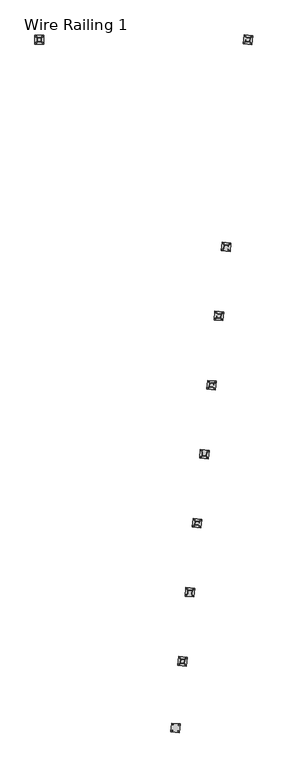
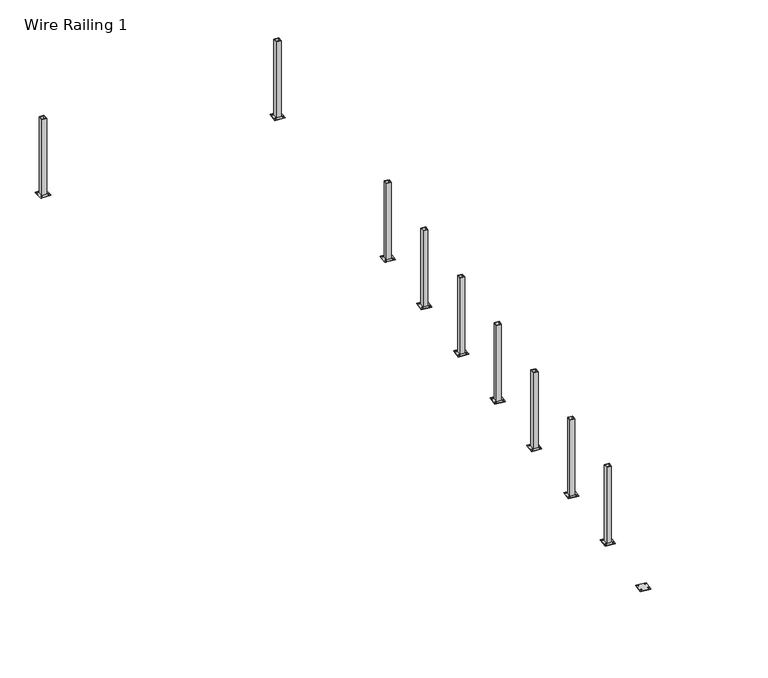
"""IFC4 building model written with IfcOpenShell, lengths in millimetres: railing geometry, Wire Railing 1."""

from ifc_helpers import new_model, si_unit, point, frame, frame_2d, origin, place, context, project, spatial, polyline, circle_curve, trimmed, segment, composite_curve, outline, extrude, source, transform, mapped, element, save


def wire_railing_1_b7aef56b(model_context):
    return source(origin(), model_context, "Body", "SweptSolid", [
        extrude(outline(composite_curve([segment(trimmed(circle_curve(frame_2d((34964.0191905, 37829.4240871)), 6.35), [point((34957.7039765, 37830.0878428))], [point((34970.3344045, 37828.7603313))], False, "CARTESIAN"), True, "CONTINUOUS"), segment(trimmed(circle_curve(frame_2d((34964.0191905, 37829.4240871)), 6.35), [point((34970.3344045, 37828.7603313))], [point((34957.7039765, 37830.0878428))], False, "CARTESIAN"), True, "CONTINUOUS")], self_intersect=False)), frame((0.0, 0.0, 269259.05), z_axis=(0.0, 0.0, 1.0), x_axis=(1.0, 0.0, 0.0)), (0.0, 0.0, 1.0), 12.7),
        extrude(outline(composite_curve([segment(trimmed(circle_curve(frame_2d((35052.432187, 37820.1315067)), 6.35), [point((35046.116973, 37820.7952624))], [point((35058.747401, 37819.4677509))], False, "CARTESIAN"), True, "CONTINUOUS"), segment(trimmed(circle_curve(frame_2d((35052.432187, 37820.1315067)), 6.35), [point((35058.747401, 37819.4677509))], [point((35046.116973, 37820.7952624))], False, "CARTESIAN"), True, "CONTINUOUS")], self_intersect=False)), frame((0.0, 0.0, 269259.05), z_axis=(0.0, 0.0, 1.0), x_axis=(1.0, 0.0, 0.0)), (0.0, 0.0, 1.0), 12.7),
        extrude(outline(composite_curve([segment(trimmed(circle_curve(frame_2d((34973.3117709, 37917.8370836)), 6.35), [point((34966.9965569, 37918.5008393))], [point((34979.6269849, 37917.1733278))], False, "CARTESIAN"), True, "CONTINUOUS"), segment(trimmed(circle_curve(frame_2d((34973.3117709, 37917.8370836)), 6.35), [point((34979.6269849, 37917.1733278))], [point((34966.9965569, 37918.5008393))], False, "CARTESIAN"), True, "CONTINUOUS")], self_intersect=False)), frame((0.0, 0.0, 269259.05), z_axis=(0.0, 0.0, 1.0), x_axis=(1.0, 0.0, 0.0)), (0.0, 0.0, 1.0), 12.7),
        extrude(outline(composite_curve([segment(trimmed(circle_curve(frame_2d((35061.7247674, 37908.5445032)), 6.35), [point((35055.4095533, 37909.2082589))], [point((35068.0399814, 37907.8807474))], False, "CARTESIAN"), True, "CONTINUOUS"), segment(trimmed(circle_curve(frame_2d((35061.7247674, 37908.5445032)), 6.35), [point((35068.0399814, 37907.8807474))], [point((35055.4095533, 37909.2082589))], False, "CARTESIAN"), True, "CONTINUOUS")], self_intersect=False)), frame((0.0, 0.0, 269259.05), z_axis=(0.0, 0.0, 1.0), x_axis=(1.0, 0.0, 0.0)), (0.0, 0.0, 1.0), 12.7),
        extrude(outline(polyline([(35069.3865619, 37799.1945973), (34943.0822812, 37812.4697122), (34956.357396, 37938.7739929), (35082.6616767, 37925.498878), (35069.3865619, 37799.1945973)])), frame((0.0, 0.0, 269259.05), z_axis=(0.0, 0.0, 1.0), x_axis=(1.0, 0.0, 0.0)), (0.0, 0.0, 1.0), 6.35),
        extrude(outline(polyline([(35039.7164058, 37835.8341887), (34979.7218725, 37842.1398682), (34986.027552, 37902.1344016), (35046.0220854, 37895.828722), (35039.7164058, 37835.8341887)]), holes=[polyline([(35034.0649475, 37842.8131584), (35039.0431156, 37890.1772637), (34991.6790103, 37895.1554318), (34986.7008423, 37847.7913265), (35034.0649475, 37842.8131584)])]), frame((0.0, 0.0, 269259.05), z_axis=(0.0, 0.0, 1.0), x_axis=(1.0, 0.0, 0.0)), (0.0, 0.0, 1.0), 1047.75),
        extrude(outline(composite_curve([segment(trimmed(circle_curve(frame_2d((34858.2648202, 36823.238465)), 6.35), [point((34851.9496061, 36823.9022208))], [point((34864.5800342, 36822.5747093))], False, "CARTESIAN"), True, "CONTINUOUS"), segment(trimmed(circle_curve(frame_2d((34858.2648202, 36823.238465)), 6.35), [point((34864.5800342, 36822.5747093))], [point((34851.9496061, 36823.9022208))], False, "CARTESIAN"), True, "CONTINUOUS")], self_intersect=False)), frame((0.0, 0.0, 269259.05), z_axis=(0.0, 0.0, 1.0), x_axis=(1.0, 0.0, 0.0)), (0.0, 0.0, 1.0), 12.7),
        extrude(outline(composite_curve([segment(trimmed(circle_curve(frame_2d((34946.6778167, 36813.9458846)), 6.35), [point((34940.3626026, 36814.6096404))], [point((34952.9930307, 36813.2821289))], False, "CARTESIAN"), True, "CONTINUOUS"), segment(trimmed(circle_curve(frame_2d((34946.6778167, 36813.9458846)), 6.35), [point((34952.9930307, 36813.2821289))], [point((34940.3626026, 36814.6096404))], False, "CARTESIAN"), True, "CONTINUOUS")], self_intersect=False)), frame((0.0, 0.0, 269259.05), z_axis=(0.0, 0.0, 1.0), x_axis=(1.0, 0.0, 0.0)), (0.0, 0.0, 1.0), 12.7),
        extrude(outline(composite_curve([segment(trimmed(circle_curve(frame_2d((34867.5574005, 36911.6514615)), 6.35), [point((34861.2421865, 36912.3152173))], [point((34873.8726146, 36910.9877058))], False, "CARTESIAN"), True, "CONTINUOUS"), segment(trimmed(circle_curve(frame_2d((34867.5574005, 36911.6514615)), 6.35), [point((34873.8726146, 36910.9877058))], [point((34861.2421865, 36912.3152173))], False, "CARTESIAN"), True, "CONTINUOUS")], self_intersect=False)), frame((0.0, 0.0, 269259.05), z_axis=(0.0, 0.0, 1.0), x_axis=(1.0, 0.0, 0.0)), (0.0, 0.0, 1.0), 12.7),
        extrude(outline(composite_curve([segment(trimmed(circle_curve(frame_2d((34955.970397, 36902.3588811)), 6.35), [point((34949.655183, 36903.0226369))], [point((34962.2856111, 36901.6951254))], False, "CARTESIAN"), True, "CONTINUOUS"), segment(trimmed(circle_curve(frame_2d((34955.970397, 36902.3588811)), 6.35), [point((34962.2856111, 36901.6951254))], [point((34949.655183, 36903.0226369))], False, "CARTESIAN"), True, "CONTINUOUS")], self_intersect=False)), frame((0.0, 0.0, 269259.05), z_axis=(0.0, 0.0, 1.0), x_axis=(1.0, 0.0, 0.0)), (0.0, 0.0, 1.0), 12.7),
        extrude(outline(polyline([(34963.6321915, 36793.0089753), (34837.3279108, 36806.2840901), (34850.6030257, 36932.5883709), (34976.9073064, 36919.313256), (34963.6321915, 36793.0089753)])), frame((0.0, 0.0, 269259.05), z_axis=(0.0, 0.0, 1.0), x_axis=(1.0, 0.0, 0.0)), (0.0, 0.0, 1.0), 6.35),
        extrude(outline(polyline([(34933.9620355, 36829.6485666), (34873.9675022, 36835.9542462), (34880.2731817, 36895.9487795), (34940.267715, 36889.6431), (34933.9620355, 36829.6485666)]), holes=[polyline([(34928.3105772, 36836.6275364), (34933.2887453, 36883.9916417), (34885.92464, 36888.9698097), (34880.9464719, 36841.6057045), (34928.3105772, 36836.6275364)])]), frame((0.0, 0.0, 269259.05), z_axis=(0.0, 0.0, 1.0), x_axis=(1.0, 0.0, 0.0)), (0.0, 0.0, 1.0), 1047.75),
        extrude(outline(composite_curve([segment(trimmed(circle_curve(frame_2d((34752.5104498, 35817.052843)), 6.35), [point((34746.1952358, 35817.7165987))], [point((34758.8256639, 35816.3890873))], False, "CARTESIAN"), True, "CONTINUOUS"), segment(trimmed(circle_curve(frame_2d((34752.5104498, 35817.052843)), 6.35), [point((34758.8256639, 35816.3890873))], [point((34746.1952358, 35817.7165987))], False, "CARTESIAN"), True, "CONTINUOUS")], self_intersect=False)), frame((0.0, 0.0, 269259.05), z_axis=(0.0, 0.0, 1.0), x_axis=(1.0, 0.0, 0.0)), (0.0, 0.0, 1.0), 12.7),
        extrude(outline(composite_curve([segment(trimmed(circle_curve(frame_2d((34840.9234463, 35807.7602626)), 6.35), [point((34834.6082323, 35808.4240184))], [point((34847.2386604, 35807.0965069))], False, "CARTESIAN"), True, "CONTINUOUS"), segment(trimmed(circle_curve(frame_2d((34840.9234463, 35807.7602626)), 6.35), [point((34847.2386604, 35807.0965069))], [point((34834.6082323, 35808.4240184))], False, "CARTESIAN"), True, "CONTINUOUS")], self_intersect=False)), frame((0.0, 0.0, 269259.05), z_axis=(0.0, 0.0, 1.0), x_axis=(1.0, 0.0, 0.0)), (0.0, 0.0, 1.0), 12.7),
        extrude(outline(composite_curve([segment(trimmed(circle_curve(frame_2d((34761.8030302, 35905.4658395)), 6.35), [point((34755.4878162, 35906.1295952))], [point((34768.1182442, 35904.8020838))], False, "CARTESIAN"), True, "CONTINUOUS"), segment(trimmed(circle_curve(frame_2d((34761.8030302, 35905.4658395)), 6.35), [point((34768.1182442, 35904.8020838))], [point((34755.4878162, 35906.1295952))], False, "CARTESIAN"), True, "CONTINUOUS")], self_intersect=False)), frame((0.0, 0.0, 269259.05), z_axis=(0.0, 0.0, 1.0), x_axis=(1.0, 0.0, 0.0)), (0.0, 0.0, 1.0), 12.7),
        extrude(outline(composite_curve([segment(trimmed(circle_curve(frame_2d((34850.2160267, 35896.1732591)), 6.35), [point((34843.9008127, 35896.8370148))], [point((34856.5312407, 35895.5095034))], False, "CARTESIAN"), True, "CONTINUOUS"), segment(trimmed(circle_curve(frame_2d((34850.2160267, 35896.1732591)), 6.35), [point((34856.5312407, 35895.5095034))], [point((34843.9008127, 35896.8370148))], False, "CARTESIAN"), True, "CONTINUOUS")], self_intersect=False)), frame((0.0, 0.0, 269259.05), z_axis=(0.0, 0.0, 1.0), x_axis=(1.0, 0.0, 0.0)), (0.0, 0.0, 1.0), 12.7),
        extrude(outline(polyline([(34857.8778212, 35786.8233533), (34731.5735405, 35800.0984681), (34744.8486553, 35926.4027488), (34871.152936, 35913.127634), (34857.8778212, 35786.8233533)])), frame((0.0, 0.0, 269259.05), z_axis=(0.0, 0.0, 1.0), x_axis=(1.0, 0.0, 0.0)), (0.0, 0.0, 1.0), 6.35),
        extrude(outline(polyline([(34828.2076652, 35823.4629446), (34768.2131318, 35829.7686242), (34774.5188114, 35889.7631575), (34834.5133447, 35883.4574779), (34828.2076652, 35823.4629446)]), holes=[polyline([(34822.5562069, 35830.4419144), (34827.5343749, 35877.8060197), (34780.1702697, 35882.7841877), (34775.1921016, 35835.4200824), (34822.5562069, 35830.4419144)])]), frame((0.0, 0.0, 269259.05), z_axis=(0.0, 0.0, 1.0), x_axis=(1.0, 0.0, 0.0)), (0.0, 0.0, 1.0), 1047.75),
        extrude(outline(composite_curve([segment(trimmed(circle_curve(frame_2d((34646.7560795, 34810.867221)), 6.35), [point((34640.4408654, 34811.5309767))], [point((34653.0712935, 34810.2034652))], False, "CARTESIAN"), True, "CONTINUOUS"), segment(trimmed(circle_curve(frame_2d((34646.7560795, 34810.867221)), 6.35), [point((34653.0712935, 34810.2034652))], [point((34640.4408654, 34811.5309767))], False, "CARTESIAN"), True, "CONTINUOUS")], self_intersect=False)), frame((0.0, 0.0, 269259.05), z_axis=(0.0, 0.0, 1.0), x_axis=(1.0, 0.0, 0.0)), (0.0, 0.0, 1.0), 12.7),
        extrude(outline(composite_curve([segment(trimmed(circle_curve(frame_2d((34735.169076, 34801.5746406)), 6.35), [point((34728.8538619, 34802.2383963))], [point((34741.48429, 34800.9108848))], False, "CARTESIAN"), True, "CONTINUOUS"), segment(trimmed(circle_curve(frame_2d((34735.169076, 34801.5746406)), 6.35), [point((34741.48429, 34800.9108848))], [point((34728.8538619, 34802.2383963))], False, "CARTESIAN"), True, "CONTINUOUS")], self_intersect=False)), frame((0.0, 0.0, 269259.05), z_axis=(0.0, 0.0, 1.0), x_axis=(1.0, 0.0, 0.0)), (0.0, 0.0, 1.0), 12.7),
        extrude(outline(composite_curve([segment(trimmed(circle_curve(frame_2d((34656.0486599, 34899.2802175)), 6.35), [point((34649.7334458, 34899.9439732))], [point((34662.3638739, 34898.6164617))], False, "CARTESIAN"), True, "CONTINUOUS"), segment(trimmed(circle_curve(frame_2d((34656.0486599, 34899.2802175)), 6.35), [point((34662.3638739, 34898.6164617))], [point((34649.7334458, 34899.9439732))], False, "CARTESIAN"), True, "CONTINUOUS")], self_intersect=False)), frame((0.0, 0.0, 269259.05), z_axis=(0.0, 0.0, 1.0), x_axis=(1.0, 0.0, 0.0)), (0.0, 0.0, 1.0), 12.7),
        extrude(outline(composite_curve([segment(trimmed(circle_curve(frame_2d((34744.4616564, 34889.9876371)), 6.35), [point((34738.1464423, 34890.6513928))], [point((34750.7768704, 34889.3238813))], False, "CARTESIAN"), True, "CONTINUOUS"), segment(trimmed(circle_curve(frame_2d((34744.4616564, 34889.9876371)), 6.35), [point((34750.7768704, 34889.3238813))], [point((34738.1464423, 34890.6513928))], False, "CARTESIAN"), True, "CONTINUOUS")], self_intersect=False)), frame((0.0, 0.0, 269259.05), z_axis=(0.0, 0.0, 1.0), x_axis=(1.0, 0.0, 0.0)), (0.0, 0.0, 1.0), 12.7),
        extrude(outline(polyline([(34752.1234509, 34780.6377312), (34625.8191702, 34793.9128461), (34639.094285, 34920.2171268), (34765.3985657, 34906.942012), (34752.1234509, 34780.6377312)])), frame((0.0, 0.0, 269259.05), z_axis=(0.0, 0.0, 1.0), x_axis=(1.0, 0.0, 0.0)), (0.0, 0.0, 1.0), 6.35),
        extrude(outline(polyline([(34722.4532948, 34817.2773226), (34662.4587615, 34823.5830021), (34668.764441, 34883.5775355), (34728.7589744, 34877.2718559), (34722.4532948, 34817.2773226)]), holes=[polyline([(34716.8018365, 34824.2562924), (34721.7800046, 34871.6203976), (34674.4158993, 34876.5985657), (34669.4377313, 34829.2344604), (34716.8018365, 34824.2562924)])]), frame((0.0, 0.0, 269259.05), z_axis=(0.0, 0.0, 1.0), x_axis=(1.0, 0.0, 0.0)), (0.0, 0.0, 1.0), 1047.75),
        extrude(outline(composite_curve([segment(trimmed(circle_curve(frame_2d((34541.0017091, 33804.6815989)), 6.35), [point((34534.6864951, 33805.3453547))], [point((34547.3169232, 33804.0178432))], False, "CARTESIAN"), True, "CONTINUOUS"), segment(trimmed(circle_curve(frame_2d((34541.0017091, 33804.6815989)), 6.35), [point((34547.3169232, 33804.0178432))], [point((34534.6864951, 33805.3453547))], False, "CARTESIAN"), True, "CONTINUOUS")], self_intersect=False)), frame((0.0, 0.0, 269259.05), z_axis=(0.0, 0.0, 1.0), x_axis=(1.0, 0.0, 0.0)), (0.0, 0.0, 1.0), 12.7),
        extrude(outline(composite_curve([segment(trimmed(circle_curve(frame_2d((34629.4147056, 33795.3890186)), 6.35), [point((34623.0994916, 33796.0527743))], [point((34635.7299197, 33794.7252628))], False, "CARTESIAN"), True, "CONTINUOUS"), segment(trimmed(circle_curve(frame_2d((34629.4147056, 33795.3890186)), 6.35), [point((34635.7299197, 33794.7252628))], [point((34623.0994916, 33796.0527743))], False, "CARTESIAN"), True, "CONTINUOUS")], self_intersect=False)), frame((0.0, 0.0, 269259.05), z_axis=(0.0, 0.0, 1.0), x_axis=(1.0, 0.0, 0.0)), (0.0, 0.0, 1.0), 12.7),
        extrude(outline(composite_curve([segment(trimmed(circle_curve(frame_2d((34550.2942895, 33893.0945954)), 6.35), [point((34543.9790755, 33893.7583512))], [point((34556.6095036, 33892.4308397))], False, "CARTESIAN"), True, "CONTINUOUS"), segment(trimmed(circle_curve(frame_2d((34550.2942895, 33893.0945954)), 6.35), [point((34556.6095036, 33892.4308397))], [point((34543.9790755, 33893.7583512))], False, "CARTESIAN"), True, "CONTINUOUS")], self_intersect=False)), frame((0.0, 0.0, 269259.05), z_axis=(0.0, 0.0, 1.0), x_axis=(1.0, 0.0, 0.0)), (0.0, 0.0, 1.0), 12.7),
        extrude(outline(composite_curve([segment(trimmed(circle_curve(frame_2d((34638.707286, 33883.802015)), 6.35), [point((34632.392072, 33884.4657708))], [point((34645.0225001, 33883.1382593))], False, "CARTESIAN"), True, "CONTINUOUS"), segment(trimmed(circle_curve(frame_2d((34638.707286, 33883.802015)), 6.35), [point((34645.0225001, 33883.1382593))], [point((34632.392072, 33884.4657708))], False, "CARTESIAN"), True, "CONTINUOUS")], self_intersect=False)), frame((0.0, 0.0, 269259.05), z_axis=(0.0, 0.0, 1.0), x_axis=(1.0, 0.0, 0.0)), (0.0, 0.0, 1.0), 12.7),
        extrude(outline(polyline([(34646.3690805, 33774.4521092), (34520.0647998, 33787.7272241), (34533.3399146, 33914.0315048), (34659.6441954, 33900.7563899), (34646.3690805, 33774.4521092)])), frame((0.0, 0.0, 269259.05), z_axis=(0.0, 0.0, 1.0), x_axis=(1.0, 0.0, 0.0)), (0.0, 0.0, 1.0), 6.35),
        extrude(outline(polyline([(34616.6989245, 33811.0917005), (34556.7043911, 33817.3973801), (34563.0100707, 33877.3919134), (34623.004604, 33871.0862339), (34616.6989245, 33811.0917005)]), holes=[polyline([(34611.0474662, 33818.0706703), (34616.0256343, 33865.4347756), (34568.661529, 33870.4129437), (34563.6833609, 33823.0488384), (34611.0474662, 33818.0706703)])]), frame((0.0, 0.0, 269259.05), z_axis=(0.0, 0.0, 1.0), x_axis=(1.0, 0.0, 0.0)), (0.0, 0.0, 1.0), 1047.75),
        extrude(outline(composite_curve([segment(trimmed(circle_curve(frame_2d((34435.2473388, 32798.4959769)), 6.35), [point((34428.9321248, 32799.1597326))], [point((34441.5625528, 32797.8322212))], False, "CARTESIAN"), True, "CONTINUOUS"), segment(trimmed(circle_curve(frame_2d((34435.2473388, 32798.4959769)), 6.35), [point((34441.5625528, 32797.8322212))], [point((34428.9321248, 32799.1597326))], False, "CARTESIAN"), True, "CONTINUOUS")], self_intersect=False)), frame((0.0, 0.0, 269259.05), z_axis=(0.0, 0.0, 1.0), x_axis=(1.0, 0.0, 0.0)), (0.0, 0.0, 1.0), 12.7),
        extrude(outline(composite_curve([segment(trimmed(circle_curve(frame_2d((34523.6603353, 32789.2033965)), 6.35), [point((34517.3451213, 32789.8671523))], [point((34529.9755493, 32788.5396408))], False, "CARTESIAN"), True, "CONTINUOUS"), segment(trimmed(circle_curve(frame_2d((34523.6603353, 32789.2033965)), 6.35), [point((34529.9755493, 32788.5396408))], [point((34517.3451213, 32789.8671523))], False, "CARTESIAN"), True, "CONTINUOUS")], self_intersect=False)), frame((0.0, 0.0, 269259.05), z_axis=(0.0, 0.0, 1.0), x_axis=(1.0, 0.0, 0.0)), (0.0, 0.0, 1.0), 12.7),
        extrude(outline(composite_curve([segment(trimmed(circle_curve(frame_2d((34444.5399192, 32886.9089734)), 6.35), [point((34438.2247052, 32887.5727291))], [point((34450.8551332, 32886.2452177))], False, "CARTESIAN"), True, "CONTINUOUS"), segment(trimmed(circle_curve(frame_2d((34444.5399192, 32886.9089734)), 6.35), [point((34450.8551332, 32886.2452177))], [point((34438.2247052, 32887.5727291))], False, "CARTESIAN"), True, "CONTINUOUS")], self_intersect=False)), frame((0.0, 0.0, 269259.05), z_axis=(0.0, 0.0, 1.0), x_axis=(1.0, 0.0, 0.0)), (0.0, 0.0, 1.0), 12.7),
        extrude(outline(composite_curve([segment(trimmed(circle_curve(frame_2d((34532.9529157, 32877.616393)), 6.35), [point((34526.6377017, 32878.2801488))], [point((34539.2681297, 32876.9526373))], False, "CARTESIAN"), True, "CONTINUOUS"), segment(trimmed(circle_curve(frame_2d((34532.9529157, 32877.616393)), 6.35), [point((34539.2681297, 32876.9526373))], [point((34526.6377017, 32878.2801488))], False, "CARTESIAN"), True, "CONTINUOUS")], self_intersect=False)), frame((0.0, 0.0, 269259.05), z_axis=(0.0, 0.0, 1.0), x_axis=(1.0, 0.0, 0.0)), (0.0, 0.0, 1.0), 12.7),
        extrude(outline(polyline([(34540.6147102, 32768.2664872), (34414.3104295, 32781.541602), (34427.5855443, 32907.8458827), (34553.889825, 32894.5707679), (34540.6147102, 32768.2664872)])), frame((0.0, 0.0, 269259.05), z_axis=(0.0, 0.0, 1.0), x_axis=(1.0, 0.0, 0.0)), (0.0, 0.0, 1.0), 6.35),
        extrude(outline(polyline([(34510.9445541, 32804.9060785), (34450.9500208, 32811.2117581), (34457.2557004, 32871.2062914), (34517.2502337, 32864.9006119), (34510.9445541, 32804.9060785)]), holes=[polyline([(34505.2930959, 32811.8850483), (34510.2712639, 32859.2491536), (34462.9071586, 32864.2273216), (34457.9289906, 32816.8632164), (34505.2930959, 32811.8850483)])]), frame((0.0, 0.0, 269259.05), z_axis=(0.0, 0.0, 1.0), x_axis=(1.0, 0.0, 0.0)), (0.0, 0.0, 1.0), 1047.75),
        extrude(outline(composite_curve([segment(trimmed(circle_curve(frame_2d((34329.4929685, 31792.3103549)), 6.35), [point((34323.1777544, 31792.9741106))], [point((34335.8081825, 31791.6465991))], False, "CARTESIAN"), True, "CONTINUOUS"), segment(trimmed(circle_curve(frame_2d((34329.4929685, 31792.3103549)), 6.35), [point((34335.8081825, 31791.6465991))], [point((34323.1777544, 31792.9741106))], False, "CARTESIAN"), True, "CONTINUOUS")], self_intersect=False)), frame((0.0, 0.0, 269259.05), z_axis=(0.0, 0.0, 1.0), x_axis=(1.0, 0.0, 0.0)), (0.0, 0.0, 1.0), 12.7),
        extrude(outline(composite_curve([segment(trimmed(circle_curve(frame_2d((34417.905965, 31783.0177745)), 6.35), [point((34411.5907509, 31783.6815302))], [point((34424.221179, 31782.3540188))], False, "CARTESIAN"), True, "CONTINUOUS"), segment(trimmed(circle_curve(frame_2d((34417.905965, 31783.0177745)), 6.35), [point((34424.221179, 31782.3540188))], [point((34411.5907509, 31783.6815302))], False, "CARTESIAN"), True, "CONTINUOUS")], self_intersect=False)), frame((0.0, 0.0, 269259.05), z_axis=(0.0, 0.0, 1.0), x_axis=(1.0, 0.0, 0.0)), (0.0, 0.0, 1.0), 12.7),
        extrude(outline(composite_curve([segment(trimmed(circle_curve(frame_2d((34338.7855489, 31880.7233514)), 6.35), [point((34332.4703348, 31881.3871071))], [point((34345.1007629, 31880.0595956))], False, "CARTESIAN"), True, "CONTINUOUS"), segment(trimmed(circle_curve(frame_2d((34338.7855489, 31880.7233514)), 6.35), [point((34345.1007629, 31880.0595956))], [point((34332.4703348, 31881.3871071))], False, "CARTESIAN"), True, "CONTINUOUS")], self_intersect=False)), frame((0.0, 0.0, 269259.05), z_axis=(0.0, 0.0, 1.0), x_axis=(1.0, 0.0, 0.0)), (0.0, 0.0, 1.0), 12.7),
        extrude(outline(composite_curve([segment(trimmed(circle_curve(frame_2d((34427.1985454, 31871.430771)), 6.35), [point((34420.8833313, 31872.0945267))], [point((34433.5137594, 31870.7670152))], False, "CARTESIAN"), True, "CONTINUOUS"), segment(trimmed(circle_curve(frame_2d((34427.1985454, 31871.430771)), 6.35), [point((34433.5137594, 31870.7670152))], [point((34420.8833313, 31872.0945267))], False, "CARTESIAN"), True, "CONTINUOUS")], self_intersect=False)), frame((0.0, 0.0, 269259.05), z_axis=(0.0, 0.0, 1.0), x_axis=(1.0, 0.0, 0.0)), (0.0, 0.0, 1.0), 12.7),
        extrude(outline(polyline([(34434.8603398, 31762.0808652), (34308.5560591, 31775.35598), (34321.831174, 31901.6602607), (34448.1354547, 31888.3851459), (34434.8603398, 31762.0808652)])), frame((0.0, 0.0, 269259.05), z_axis=(0.0, 0.0, 1.0), x_axis=(1.0, 0.0, 0.0)), (0.0, 0.0, 1.0), 6.35),
        extrude(outline(polyline([(34405.1901838, 31798.7204565), (34345.1956505, 31805.026136), (34351.50133, 31865.0206694), (34411.4958634, 31858.7149898), (34405.1901838, 31798.7204565)]), holes=[polyline([(34399.5387255, 31805.6994263), (34404.5168936, 31853.0635315), (34357.1527883, 31858.0416996), (34352.1746202, 31810.6775943), (34399.5387255, 31805.6994263)])]), frame((0.0, 0.0, 269259.05), z_axis=(0.0, 0.0, 1.0), x_axis=(1.0, 0.0, 0.0)), (0.0, 0.0, 1.0), 1047.75),
        extrude(outline(composite_curve([segment(trimmed(circle_curve(frame_2d((35281.2823015, 40847.9809531)), 6.35), [point((35274.9670875, 40848.6447089))], [point((35287.5975156, 40847.3171974))], False, "CARTESIAN"), True, "CONTINUOUS"), segment(trimmed(circle_curve(frame_2d((35281.2823015, 40847.9809531)), 6.35), [point((35287.5975156, 40847.3171974))], [point((35274.9670875, 40848.6447089))], False, "CARTESIAN"), True, "CONTINUOUS")], self_intersect=False)), frame((0.0, 0.0, 269259.05), z_axis=(0.0, 0.0, 1.0), x_axis=(1.0, 0.0, 0.0)), (0.0, 0.0, 1.0), 12.7),
        extrude(outline(composite_curve([segment(trimmed(circle_curve(frame_2d((35369.695298, 40838.6883728)), 6.35), [point((35363.380084, 40839.3521285))], [point((35376.0105121, 40838.024617))], False, "CARTESIAN"), True, "CONTINUOUS"), segment(trimmed(circle_curve(frame_2d((35369.695298, 40838.6883728)), 6.35), [point((35376.0105121, 40838.024617))], [point((35363.380084, 40839.3521285))], False, "CARTESIAN"), True, "CONTINUOUS")], self_intersect=False)), frame((0.0, 0.0, 269259.05), z_axis=(0.0, 0.0, 1.0), x_axis=(1.0, 0.0, 0.0)), (0.0, 0.0, 1.0), 12.7),
        extrude(outline(composite_curve([segment(trimmed(circle_curve(frame_2d((35290.5748819, 40936.3939496)), 6.35), [point((35284.2596679, 40937.0577054))], [point((35296.8900959, 40935.7301939))], False, "CARTESIAN"), True, "CONTINUOUS"), segment(trimmed(circle_curve(frame_2d((35290.5748819, 40936.3939496)), 6.35), [point((35296.8900959, 40935.7301939))], [point((35284.2596679, 40937.0577054))], False, "CARTESIAN"), True, "CONTINUOUS")], self_intersect=False)), frame((0.0, 0.0, 269259.05), z_axis=(0.0, 0.0, 1.0), x_axis=(1.0, 0.0, 0.0)), (0.0, 0.0, 1.0), 12.7),
        extrude(outline(composite_curve([segment(trimmed(circle_curve(frame_2d((35378.9878784, 40927.1013693)), 6.35), [point((35372.6726644, 40927.765125))], [point((35385.3030924, 40926.4376135))], False, "CARTESIAN"), True, "CONTINUOUS"), segment(trimmed(circle_curve(frame_2d((35378.9878784, 40927.1013693)), 6.35), [point((35385.3030924, 40926.4376135))], [point((35372.6726644, 40927.765125))], False, "CARTESIAN"), True, "CONTINUOUS")], self_intersect=False)), frame((0.0, 0.0, 269259.05), z_axis=(0.0, 0.0, 1.0), x_axis=(1.0, 0.0, 0.0)), (0.0, 0.0, 1.0), 12.7),
        extrude(outline(polyline([(35386.6496729, 40817.7514634), (35260.3453922, 40831.0265783), (35273.620507, 40957.330859), (35399.9247877, 40944.0557441), (35386.6496729, 40817.7514634)])), frame((0.0, 0.0, 269259.05), z_axis=(0.0, 0.0, 1.0), x_axis=(1.0, 0.0, 0.0)), (0.0, 0.0, 1.0), 6.35),
        extrude(outline(polyline([(35356.9795169, 40854.3910548), (35296.9849835, 40860.6967343), (35303.2906631, 40920.6912676), (35363.2851964, 40914.3855881), (35356.9795169, 40854.3910548)]), holes=[polyline([(35351.3280586, 40861.3700245), (35356.3062266, 40908.7341298), (35308.9421214, 40913.7122979), (35303.9639533, 40866.3481926), (35351.3280586, 40861.3700245)])]), frame((0.0, 0.0, 269259.05), z_axis=(0.0, 0.0, 1.0), x_axis=(1.0, 0.0, 0.0)), (0.0, 0.0, 1.0), 1047.75),
        extrude(outline(composite_curve([segment(trimmed(circle_curve(frame_2d((32337.1627201, 40843.0911612)), 6.35), [point((32337.1627201, 40836.7411612))], [point((32337.1627201, 40849.4411612))], False, "CARTESIAN"), True, "CONTINUOUS"), segment(trimmed(circle_curve(frame_2d((32337.1627201, 40843.0911612)), 6.35), [point((32337.1627201, 40849.4411612))], [point((32337.1627201, 40836.7411612))], False, "CARTESIAN"), True, "CONTINUOUS")], self_intersect=False)), frame((0.0, 0.0, 269259.05), z_axis=(0.0, 0.0, 1.0), x_axis=(1.0, 0.0, 0.0)), (0.0, 0.0, 1.0), 12.7),
        extrude(outline(composite_curve([segment(trimmed(circle_curve(frame_2d((32337.1627201, 40931.9911612)), 6.35), [point((32337.1627201, 40925.6411612))], [point((32337.1627201, 40938.3411612))], False, "CARTESIAN"), True, "CONTINUOUS"), segment(trimmed(circle_curve(frame_2d((32337.1627201, 40931.9911612)), 6.35), [point((32337.1627201, 40938.3411612))], [point((32337.1627201, 40925.6411612))], False, "CARTESIAN"), True, "CONTINUOUS")], self_intersect=False)), frame((0.0, 0.0, 269259.05), z_axis=(0.0, 0.0, 1.0), x_axis=(1.0, 0.0, 0.0)), (0.0, 0.0, 1.0), 12.7),
        extrude(outline(composite_curve([segment(trimmed(circle_curve(frame_2d((32248.2627201, 40843.0911612)), 6.35), [point((32248.2627201, 40836.7411612))], [point((32248.2627201, 40849.4411612))], False, "CARTESIAN"), True, "CONTINUOUS"), segment(trimmed(circle_curve(frame_2d((32248.2627201, 40843.0911612)), 6.35), [point((32248.2627201, 40849.4411612))], [point((32248.2627201, 40836.7411612))], False, "CARTESIAN"), True, "CONTINUOUS")], self_intersect=False)), frame((0.0, 0.0, 269259.05), z_axis=(0.0, 0.0, 1.0), x_axis=(1.0, 0.0, 0.0)), (0.0, 0.0, 1.0), 12.7),
        extrude(outline(composite_curve([segment(trimmed(circle_curve(frame_2d((32248.2627201, 40931.9911612)), 6.35), [point((32248.2627201, 40925.6411612))], [point((32248.2627201, 40938.3411612))], False, "CARTESIAN"), True, "CONTINUOUS"), segment(trimmed(circle_curve(frame_2d((32248.2627201, 40931.9911612)), 6.35), [point((32248.2627201, 40938.3411612))], [point((32248.2627201, 40925.6411612))], False, "CARTESIAN"), True, "CONTINUOUS")], self_intersect=False)), frame((0.0, 0.0, 269259.05), z_axis=(0.0, 0.0, 1.0), x_axis=(1.0, 0.0, 0.0)), (0.0, 0.0, 1.0), 12.7),
        extrude(outline(polyline([(32356.2127201, 40951.0411612), (32356.2127201, 40824.0411612), (32229.2127201, 40824.0411612), (32229.2127201, 40951.0411612), (32356.2127201, 40951.0411612)])), frame((0.0, 0.0, 269259.05), z_axis=(0.0, 0.0, 1.0), x_axis=(1.0, 0.0, 0.0)), (0.0, 0.0, 1.0), 6.35),
        extrude(outline(polyline([(32322.8752201, 40917.7036612), (32322.8752201, 40857.3786612), (32262.5502201, 40857.3786612), (32262.5502201, 40917.7036612), (32322.8752201, 40917.7036612)]), holes=[polyline([(32316.5252201, 40911.3536612), (32268.9002201, 40911.3536612), (32268.9002201, 40863.7286612), (32316.5252201, 40863.7286612), (32316.5252201, 40911.3536612)])]), frame((0.0, 0.0, 269259.05), z_axis=(0.0, 0.0, 1.0), x_axis=(1.0, 0.0, 0.0)), (0.0, 0.0, 1.0), 1047.75),
        extrude(outline(composite_curve([segment(trimmed(circle_curve(frame_2d((34227.7211326, 30824.0160171)), 6.35), [point((34221.4059185, 30824.6797728))], [point((34234.0363466, 30823.3522613))], False, "CARTESIAN"), True, "CONTINUOUS"), segment(trimmed(circle_curve(frame_2d((34227.7211326, 30824.0160171)), 6.35), [point((34234.0363466, 30823.3522613))], [point((34221.4059185, 30824.6797728))], False, "CARTESIAN"), True, "CONTINUOUS")], self_intersect=False)), frame((0.0, 0.0, 269259.05), z_axis=(0.0, 0.0, 1.0), x_axis=(1.0, 0.0, 0.0)), (0.0, 0.0, 1.0), 12.7),
        extrude(outline(composite_curve([segment(trimmed(circle_curve(frame_2d((34316.1341291, 30814.7234367)), 6.35), [point((34309.818915, 30815.3871924))], [point((34322.4493431, 30814.0596809))], False, "CARTESIAN"), True, "CONTINUOUS"), segment(trimmed(circle_curve(frame_2d((34316.1341291, 30814.7234367)), 6.35), [point((34322.4493431, 30814.0596809))], [point((34309.818915, 30815.3871924))], False, "CARTESIAN"), True, "CONTINUOUS")], self_intersect=False)), frame((0.0, 0.0, 269259.05), z_axis=(0.0, 0.0, 1.0), x_axis=(1.0, 0.0, 0.0)), (0.0, 0.0, 1.0), 12.7),
        extrude(outline(composite_curve([segment(trimmed(circle_curve(frame_2d((34237.013713, 30912.4290136)), 6.35), [point((34230.6984989, 30913.0927693))], [point((34243.328927, 30911.7652578))], False, "CARTESIAN"), True, "CONTINUOUS"), segment(trimmed(circle_curve(frame_2d((34237.013713, 30912.4290136)), 6.35), [point((34243.328927, 30911.7652578))], [point((34230.6984989, 30913.0927693))], False, "CARTESIAN"), True, "CONTINUOUS")], self_intersect=False)), frame((0.0, 0.0, 269259.05), z_axis=(0.0, 0.0, 1.0), x_axis=(1.0, 0.0, 0.0)), (0.0, 0.0, 1.0), 12.7),
        extrude(outline(composite_curve([segment(trimmed(circle_curve(frame_2d((34325.4267095, 30903.1364332)), 6.35), [point((34319.1114954, 30903.8001889))], [point((34331.7419235, 30902.4726774))], False, "CARTESIAN"), True, "CONTINUOUS"), segment(trimmed(circle_curve(frame_2d((34325.4267095, 30903.1364332)), 6.35), [point((34331.7419235, 30902.4726774))], [point((34319.1114954, 30903.8001889))], False, "CARTESIAN"), True, "CONTINUOUS")], self_intersect=False)), frame((0.0, 0.0, 269259.05), z_axis=(0.0, 0.0, 1.0), x_axis=(1.0, 0.0, 0.0)), (0.0, 0.0, 1.0), 12.7),
        extrude(outline(polyline([(34333.088504, 30793.7865273), (34206.7842232, 30807.0616422), (34220.0593381, 30933.3659229), (34346.3636188, 30920.0908081), (34333.088504, 30793.7865273)])), frame((0.0, 0.0, 269259.05), z_axis=(0.0, 0.0, 1.0), x_axis=(1.0, 0.0, 0.0)), (0.0, 0.0, 1.0), 6.35),
    ])


if __name__ == "__main__":
    model = new_model("IFC4")
    model_context = context("Model", 3, world=origin())
    ifc_project = project(units=[si_unit("LENGTHUNIT", "METRE", prefix="MILLI")], contexts=[model_context])
    site = spatial("IfcSite", under=ifc_project)
    building = spatial("IfcBuilding", under=site)
    placement = place(None, origin())
    wire_railing_1_shape = wire_railing_1_b7aef56b(model_context)
    element("IfcRailing", 1, ObjectType="Wire Railing 1", at=placement, inside=building, context=model_context, shape_type="MappedRepresentation", body=[
        mapped(wire_railing_1_shape, transform((0.0, 0.0, 0.0), x_axis=(1.0, 0.0, 0.0), y_axis=(0.0, 1.0, 0.0), z_axis=(0.0, 0.0, 1.0))),
    ])
    save(model, "model.ifc")

# Revit data of these elements
# Element 1 (IfcRailing, "Wire Railing 1")
#   Materials on its faces: "WIRE RAILING"
# Materials
#   "WIRE RAILING": class "Metal", colour RGB 244 244 244, transparency 0, Manufacturer = "Kawneer", URL = "http://www.kawneer.com/kawneer/north_america/en/home.asp", Cost = 0
